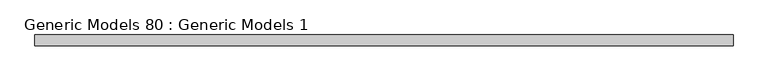
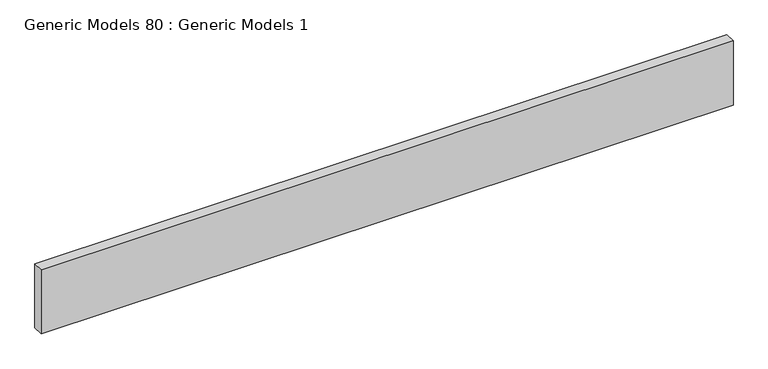
"""IFC4 building model written with IfcOpenShell, lengths in millimetres: proxy geometry, Generic Models 80 : Generic Models 1."""

import ifcopenshell
import ifcopenshell.guid

model = None  # the IFC model being written
_history = None  # IfcOwnerHistory: only IFC2X3 demands one
_inside = {}  # id of a spatial element -> (the spatial element, [elements in it])
_under = {}  # id of a project, library or spatial element -> (it, [spatial elements below it])
_declared = {}  # id of a project -> (the project, [libraries it declares])
_typed = {}  # id of a type object -> (the type object, [elements of that type])
_made_of = {}  # id of a material, layer set ... -> (it, [elements and type objects made of it])


def new_model(schema):
    """Start an empty IFC model of exactly this schema.

    Asked for "IFC4X3", IfcOpenShell would pick the latest addendum, in which some entities
    have other attributes; the version numbers below select the first issue.
    IFC2X3 requires an IfcOwnerHistory on every rooted entity: one is made here for all.
    """
    global model, _history
    if schema == "IFC4X3":
        model = ifcopenshell.file(schema_version=(4, 3, 0, 0))
    else:
        model = ifcopenshell.file(schema=schema)
    _inside.clear()
    _under.clear()
    _declared.clear()
    _typed.clear()
    _made_of.clear()
    _history = None
    if model.schema == "IFC2X3":
        org = make("IfcOrganization", Name="unknown")
        user = make(
            "IfcPersonAndOrganization",
            ThePerson=make("IfcPerson", FamilyName="unknown"),
            TheOrganization=org,
        )
        app = make(
            "IfcApplication",
            ApplicationDeveloper=org,
            Version="unknown",
            ApplicationFullName="unknown",
            ApplicationIdentifier="unknown",
        )
        _history = make(
            "IfcOwnerHistory",
            OwningUser=user,
            OwningApplication=app,
            ChangeAction="ADDED",
            CreationDate=0,
        )
    return model


def make(cls, **values):
    """One entity of the class cls with the attributes given. An attribute that is None is left unset."""
    return model.create_entity(
        cls, **{name: value for name, value in values.items() if value is not None}
    )


def rooted(cls, **values):
    """An entity with a GlobalId (a new one), such as an element, a storey or a relation."""
    return make(cls, GlobalId=ifcopenshell.guid.new(), OwnerHistory=_history, **values)


def si_unit(unit_type, name, prefix=None):
    """IfcSIUnit, for example si_unit("LENGTHUNIT", "METRE", prefix="MILLI")."""
    return make("IfcSIUnit", UnitType=unit_type, Prefix=prefix, Name=name)


def assignment(units):
    """IfcUnitAssignment: the units of a project."""
    return None if units is None else make("IfcUnitAssignment", Units=units)


def point(xyz):
    """IfcCartesianPoint."""
    return None if xyz is None else make("IfcCartesianPoint", Coordinates=xyz)


def direction(xyz):
    """IfcDirection."""
    return None if xyz is None else make("IfcDirection", DirectionRatios=xyz)


def frame(location, z_axis=None, x_axis=None):
    """IfcAxis2Placement3D, a coordinate frame: its origin and axes. An axis left out is left unset."""
    return make(
        "IfcAxis2Placement3D",
        Location=point(location),
        Axis=direction(z_axis),
        RefDirection=direction(x_axis),
    )


def origin():
    """The frame at (0, 0, 0) with its axes left unset."""
    return frame((0.0, 0.0, 0.0))


def place(relative_to, where):
    """IfcLocalPlacement: puts the frame where relative to a parent placement (None: the world)."""
    return make(
        "IfcLocalPlacement", PlacementRelTo=relative_to, RelativePlacement=where
    )


def context(
    kind, dimensions, precision=None, world=None, true_north=None, identifier=None
):
    """IfcGeometricRepresentationContext, for example the 3D "Model" context."""
    return make(
        "IfcGeometricRepresentationContext",
        ContextIdentifier=identifier,
        ContextType=kind,
        CoordinateSpaceDimension=dimensions,
        Precision=precision,
        WorldCoordinateSystem=world,
        TrueNorth=true_north,
    )


def project(units=None, contexts=None):
    """IfcProject with its units and contexts."""
    return rooted(
        "IfcProject",
        Name="project",
        RepresentationContexts=contexts,
        UnitsInContext=assignment(units),
    )


def spatial(cls, under=None, at=None, **own):
    """A site, building, storey or space (cls), placed at a placement, below another one or the project."""
    s = rooted(cls, ObjectPlacement=at, **own)
    if under is not None:
        _under.setdefault(under.id(), (under, []))[1].append(s)
    return s


def polyline(points):
    """IfcPolyline through the points."""
    return make("IfcPolyline", Points=[point(p) for p in points])


def outline(outer, holes=None, kind="AREA"):
    """IfcArbitraryClosedProfileDef: a profile drawn as a closed curve; with holes, ...WithVoids."""
    if holes is None:
        return make("IfcArbitraryClosedProfileDef", ProfileType=kind, OuterCurve=outer)
    return make(
        "IfcArbitraryProfileDefWithVoids",
        ProfileType=kind,
        OuterCurve=outer,
        InnerCurves=holes,
    )


def extrude(swept, where, along, depth):
    """IfcExtrudedAreaSolid: the profile swept, set in the frame where, extruded along a direction by depth."""
    return make(
        "IfcExtrudedAreaSolid",
        SweptArea=swept,
        Position=where,
        ExtrudedDirection=direction(along),
        Depth=depth,
    )


def shape(context_of_items, identifier, shape_type, items):
    """IfcShapeRepresentation: the items that make up one representation, for example the "Body"."""
    return make(
        "IfcShapeRepresentation",
        ContextOfItems=context_of_items,
        RepresentationIdentifier=identifier,
        RepresentationType=shape_type,
        Items=items,
    )


def source(mapping_origin, context_of_items, identifier, shape_type, items):
    """IfcRepresentationMap: a shape defined once, which mapped items show again and again."""
    return make(
        "IfcRepresentationMap",
        MappingOrigin=mapping_origin,
        MappedRepresentation=shape(context_of_items, identifier, shape_type, items),
    )


def transform(
    local_origin,
    x_axis=None,
    y_axis=None,
    z_axis=None,
    scale=None,
    scale2=None,
    scale3=None,
    uniform=True,
):
    """IfcCartesianTransformationOperator3D, or its non-uniform kind. x_axis, y_axis, z_axis: its Axis1, 2, 3."""
    if uniform:
        return make(
            "IfcCartesianTransformationOperator3D",
            Axis1=direction(x_axis),
            Axis2=direction(y_axis),
            LocalOrigin=point(local_origin),
            Scale=scale,
            Axis3=direction(z_axis),
        )
    return make(
        "IfcCartesianTransformationOperator3DnonUniform",
        Axis1=direction(x_axis),
        Axis2=direction(y_axis),
        LocalOrigin=point(local_origin),
        Scale=scale,
        Axis3=direction(z_axis),
        Scale2=scale2,
        Scale3=scale3,
    )


def mapped(mapping_source, mapping_target):
    """IfcMappedItem: shows the shape of a source again, moved by a transform."""
    return make(
        "IfcMappedItem", MappingSource=mapping_source, MappingTarget=mapping_target
    )


def made_of(thing, what):
    """Note that an element or type object is made of a material, layer set ...; save() writes the relation."""
    if what is not None:
        _made_of.setdefault(what.id(), (what, []))[1].append(thing)
    return thing


def element(
    cls,
    number,
    at=None,
    inside=None,
    cuts=None,
    type_object=None,
    material=None,
    context=None,
    identifier="Body",
    shape_type=None,
    held_by="IfcProductDefinitionShape",
    body=None,
    shapes=None,
    **own,
):
    """One element of the class cls, such as IfcWall. Its Tag is "e" and its number.

    at: its placement. inside: the storey or other place that contains it. cuts: it is an
    opening in that element (IfcRelVoidsElement). A single representation is given by context,
    identifier, shape_type and body (its items); several are given by shapes. held_by: the class
    of the entity that holds the representations. save() writes the other relations.
    """
    e = rooted(cls, Tag="e%d" % number, ObjectPlacement=at, **own)
    if body is not None:
        shapes = [shape(context, identifier, shape_type, body)]
    if shapes is not None:
        e.Representation = make(held_by, Representations=shapes)
    if inside is not None:
        _inside.setdefault(inside.id(), (inside, []))[1].append(e)
    if cuts is not None:
        rooted(
            "IfcRelVoidsElement", RelatingBuildingElement=cuts, RelatedOpeningElement=e
        )
    if type_object is not None:
        _typed.setdefault(type_object.id(), (type_object, []))[1].append(e)
    return made_of(e, material)


def aggregate(whole, parts):
    """IfcRelAggregates: a whole, such as a stair, and the parts it consists of."""
    return rooted("IfcRelAggregates", RelatingObject=whole, RelatedObjects=parts)


def save(model, path):
    """Write the relations noted so far, then the file.

    IfcRelAggregates (storeys below a building ...), IfcRelContainedInSpatialStructure (elements
    in a storey), IfcRelDefinesByType, IfcRelAssociatesMaterial and IfcRelDeclares: one each for
    every whole, place, type object, material and project.
    """
    for whole, parts in _under.values():
        aggregate(whole, parts)
    for where, things in _inside.values():
        rooted(
            "IfcRelContainedInSpatialStructure",
            RelatedElements=things,
            RelatingStructure=where,
        )
    for kind, things in _typed.values():
        rooted("IfcRelDefinesByType", RelatedObjects=things, RelatingType=kind)
    for what, things in _made_of.values():
        rooted("IfcRelAssociatesMaterial", RelatedObjects=things, RelatingMaterial=what)
    for by, libraries in _declared.values():
        rooted("IfcRelDeclares", RelatingContext=by, RelatedDefinitions=libraries)
    model.write(path)


def generic_models_80_generic_models_1_0721b936(model_context):
    return source(origin(), model_context, "Body", "SweptSolid", [
        extrude(outline(polyline([(-5091.6036296, 497.8977803), (-5091.6036296, 542.3477803), (-2183.3036295, 542.3477803), (-2183.3036295, 497.8977803), (-5091.6036296, 497.8977803)])), frame((0.0, 0.0, 126485.396), z_axis=(0.0, 0.0, 1.0), x_axis=(1.0, 0.0, 0.0)), (0.0, 0.0, 1.0), 285.75),
    ])


if __name__ == "__main__":
    model = new_model("IFC4")
    model_context = context("Model", 3, world=origin())
    ifc_project = project(units=[si_unit("LENGTHUNIT", "METRE", prefix="MILLI")], contexts=[model_context])
    site = spatial("IfcSite", under=ifc_project)
    building = spatial("IfcBuilding", under=site)
    placement = place(None, origin())
    generic_models_80_generic_models_1_shape = generic_models_80_generic_models_1_0721b936(model_context)
    element("IfcBuildingElementProxy", 1, Name="Generic Models 80 : Generic Models 1", ObjectType="Generic Models 80 : Generic Models 1", at=placement, inside=building, context=model_context, shape_type="MappedRepresentation", body=[
        mapped(generic_models_80_generic_models_1_shape, transform((0.0, 0.0, 0.0), x_axis=(1.0, 0.0, 0.0), y_axis=(0.0, 1.0, 0.0), z_axis=(0.0, 0.0, 1.0))),
    ])
    save(model, "model.ifc")

# Revit data of these elements
# Element 1 (IfcBuildingElementProxy, "Generic Models 80 : Generic Models 1")
#   Materials on its faces: "_STRUCTURAL MEMBER (SEE STRUCT. DWGS)"
# Materials
#   "_STRUCTURAL MEMBER (SEE STRUCT. DWGS)": class "Generic", colour RGB 209 182 141, transparency 0, Cost = 0
